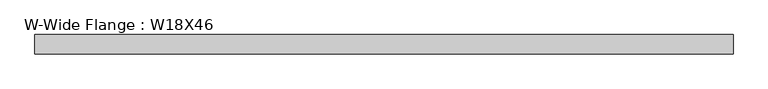
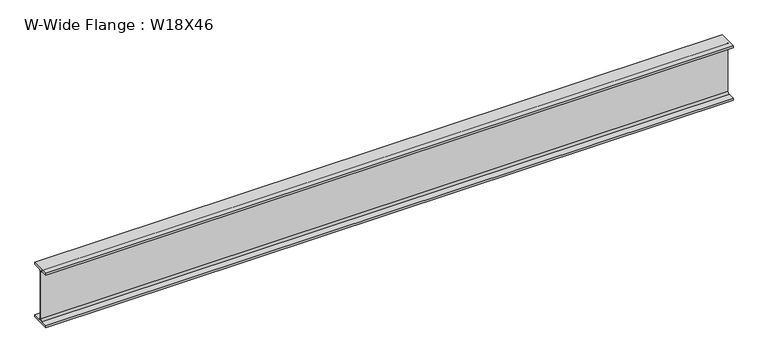
"""IFC4 building model written with IfcOpenShell, lengths in millimetres: beam geometry, W-Wide Flange : W18X46."""

from ifc_helpers import new_model, si_unit, point, frame, frame_2d, origin, place, context, project, spatial, polyline, circle_curve, trimmed, segment, composite_curve, outline, extrude, source, transform, mapped, element, save


def w_wide_flange_w18x46_4d9f21ed(model_context):
    return source(origin(), model_context, "Body", "SweptSolid", [
        extrude(outline(composite_curve([segment(polyline([(76.962, -214.503), (76.962, -229.87), (-76.962, -229.87), (-76.962, -214.503), (-20.955, -214.503)]), True, "CONTINUOUS"), segment(trimmed(circle_curve(frame_2d((-20.955, -198.12)), 16.383), [point((-20.955, -214.503))], [point((-4.572, -198.12))], True, "CARTESIAN"), True, "CONTINUOUS"), segment(polyline([(-4.572, -198.12), (-4.572, 198.12)]), True, "CONTINUOUS"), segment(trimmed(circle_curve(frame_2d((-20.955, 198.12)), 16.383), [point((-4.572, 198.12))], [point((-20.955, 214.503))], True, "CARTESIAN"), True, "CONTINUOUS"), segment(polyline([(-20.955, 214.503), (-76.962, 214.503), (-76.962, 229.87), (76.962, 229.87), (76.962, 214.503), (20.955, 214.503)]), True, "CONTINUOUS"), segment(trimmed(circle_curve(frame_2d((20.955, 198.12)), 16.383), [point((20.955, 214.503))], [point((4.572, 198.12))], True, "CARTESIAN"), True, "CONTINUOUS"), segment(polyline([(4.572, 198.12), (4.572, -198.12)]), True, "CONTINUOUS"), segment(trimmed(circle_curve(frame_2d((20.955, -198.12)), 16.383), [point((4.572, -198.12))], [point((20.955, -214.503))], True, "CARTESIAN"), True, "CONTINUOUS"), segment(polyline([(20.955, -214.503), (76.962, -214.503)]), True, "CONTINUOUS")], self_intersect=False)), frame((-2755.9, 0.0, 0.0), z_axis=(1.0, 0.0, 0.0), x_axis=(0.0, 1.0, 0.0)), (0.0, 0.0, 1.0), 5511.8),
    ])


if __name__ == "__main__":
    model = new_model("IFC4")
    model_context = context("Model", 3, world=origin())
    ifc_project = project(units=[si_unit("LENGTHUNIT", "METRE", prefix="MILLI")], contexts=[model_context])
    site = spatial("IfcSite", under=ifc_project)
    building = spatial("IfcBuilding", under=site)
    placement = place(None, origin())
    w_wide_flange_w18x46_shape = w_wide_flange_w18x46_4d9f21ed(model_context)
    element("IfcBeam", 1, ObjectType="W-Wide Flange : W18X46", at=placement, inside=building, context=model_context, shape_type="MappedRepresentation", body=[
        mapped(w_wide_flange_w18x46_shape, transform((0.0, 0.0, 0.0), x_axis=(1.0, 0.0, 0.0), y_axis=(0.0, 1.0, 0.0), z_axis=(0.0, 0.0, 1.0))),
    ])
    save(model, "model.ifc")

# Revit data of these elements
# Type "W-Wide Flange : W18X46"
#   Assembly Code = "B10"
#   W = 46
#   Length [instance default] = 5' - 0"
#   bf = 0' - 6.06"
#   d = 1' - 6.1"
#   k = 0' - 1 1/4"
#   k2 = 0' - 0.645"
#   tf = 0' - 0.605"
#   tw = 0' - 0.36"
#   A = 0.09375 SF
#   Structural Material [instance default] = Steel ASTM A992
# Element 1 (IfcBeam, "W-Wide Flange : W18X46")
#   Materials on its faces: "Steel ASTM A992"
# Materials
#   "Steel ASTM A992": class "Metal", colour RGB 199 199 199, transparency 0, Description = "Structural steel 50ksi", Cost = 0
